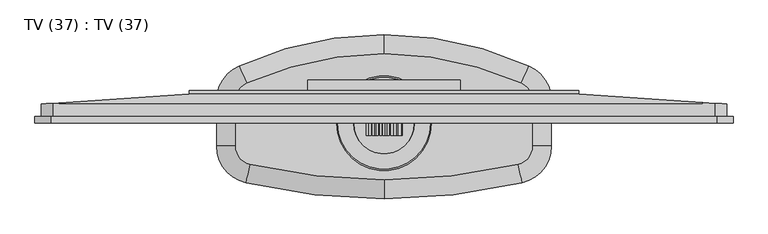
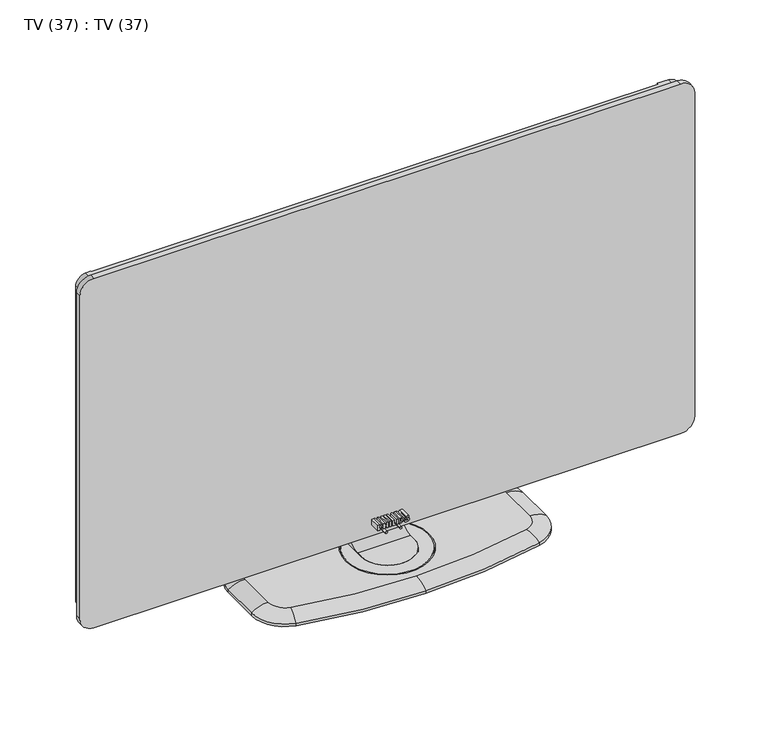
"""IFC4 building model written with IfcOpenShell, lengths in millimetres: furniture geometry, TV (37) : TV (37)."""

from ifc_helpers import new_model, si_unit, point, frame, frame_2d, origin, place, context, project, spatial, polyline, circle_curve, ellipse_curve, trimmed, segment, composite_curve, outline, extrude, source, transform, mapped, element, save
from ifc_brep_helpers import plane_surface, cylinder_surface, revolved_surface, advanced_brep


def tv_37_tv_37_55a44b14(model_context):
    return source(origin(), model_context, "Body", "SolidModel", [
        advanced_brep(
        [(47.5, 88.0, 133.1843541), (47.5, 88.0, 218.1843541), (47.5, 78.0, 218.1843541), (47.5, 78.0, 133.6678583), (47.5, 59.7827761, 41.2895959), (47.5, 32.0312094, 20.0814552), (47.5, 29.7558767, 20.0), (47.5, 18.8623336, 20.0), (47.5, 18.8623336, 10.0), (47.5, 44.5, 10.0), (47.5, 69.2193203, 37.9802704), (-47.5, 88.0, 133.1843541), (-47.5, 69.2193203, 37.9802704), (-47.5, 44.5, 10.0), (-47.5, 18.8623336, 10.0), (-47.5, 18.8623336, 20.0), (-47.5, 29.7558767, 20.0), (-47.5, 32.0312094, 20.0814552), (-47.5, 59.7827761, 41.2895959), (-47.5, 78.0, 133.6678583), (-47.5, 78.0, 218.1843541), (-47.5, 88.0, 218.1843541)],
        [
            (0, 1),
            (1, 2),
            (2, 3),
            (3, 4, circle_curve(frame((47.5, -252.8458142, 150.9261062), z_axis=(-1.0, 0.0, 0.0), x_axis=(0.0, 1.0, 0.0)), 331.2956382)),
            (4, 5, circle_curve(frame((47.5, 29.7558767, 51.8198052), z_axis=(-1.0, 0.0, 0.0), x_axis=(0.0, 1.0, 0.0)), 31.8198052)),
            (5, 6, circle_curve(frame((47.5, 29.7558767, 51.8198052), z_axis=(-1.0, 0.0, 0.0), x_axis=(0.0, 1.0, 0.0)), 31.8198052)),
            (6, 7),
            (7, 8),
            (8, 9),
            (9, 10, circle_curve(frame((47.5, 16.5507824, 59.6012298), z_axis=(1.0, 0.0, 0.0), x_axis=(0.0, 1.0, 0.0)), 56.9336523)),
            (10, 0, circle_curve(frame((47.5, -162.6973021, 133.1843541), z_axis=(1.0, 0.0, 0.0), x_axis=(0.0, 1.0, 0.0)), 250.6973021)),
            (11, 12, circle_curve(frame((-47.5, -162.6973021, 133.1843541), z_axis=(-1.0, 0.0, 0.0), x_axis=(0.0, 1.0, 0.0)), 250.6973021)),
            (12, 13, circle_curve(frame((-47.5, 16.5507824, 59.6012298), z_axis=(-1.0, 0.0, 0.0), x_axis=(0.0, 1.0, 0.0)), 56.9336523)),
            (13, 14),
            (14, 15),
            (15, 16),
            (16, 17, circle_curve(frame((-47.5, 29.7558767, 51.8198052), z_axis=(1.0, 0.0, 0.0), x_axis=(0.0, 1.0, 0.0)), 31.8198052)),
            (17, 18, circle_curve(frame((-47.5, 29.7558767, 51.8198052), z_axis=(1.0, 0.0, 0.0), x_axis=(0.0, 1.0, 0.0)), 31.8198052)),
            (18, 19, circle_curve(frame((-47.5, -252.8458142, 150.9261062), z_axis=(1.0, 0.0, 0.0), x_axis=(0.0, 1.0, 0.0)), 331.2956382)),
            (19, 20),
            (20, 21),
            (21, 11),
            (0, 11),
            (21, 1),
            (20, 2),
            (19, 3),
            (18, 4),
            (16, 6),
            (15, 7, circle_curve(frame((0.0, 18.8623336, 20.0), z_axis=(0.0, 0.0, 1.0), x_axis=(1.0, 0.0, 0.0)), 47.5)),
            (8, 14, circle_curve(frame((0.0, 18.8623336, 10.0), z_axis=(0.0, 0.0, -1.0), x_axis=(1.0, 0.0, 0.0)), 47.5)),
            (13, 9),
            (12, 10),
        ],
        [
            plane_surface(frame((47.5, 88.0, 393.1843541), z_axis=(1.0, 0.0, 0.0), x_axis=(0.0, 0.0, 1.0))),
            plane_surface(frame((-47.5, 88.0, 393.1843541), z_axis=(-1.0, 0.0, 0.0), x_axis=(0.0, 0.0, -1.0))),
            plane_surface(frame((47.5, 88.0, 133.1843541), z_axis=(0.0, 1.0, 0.0), x_axis=(-1.0, 0.0, 0.0))),
            plane_surface(frame((47.5, 88.0, 218.1843541), z_axis=(0.0, 0.0, 1.0), x_axis=(-1.0, 0.0, 0.0))),
            plane_surface(frame((47.5, 78.0, 218.1843541), z_axis=(0.0, -1.0, 0.0), x_axis=(-1.0, 0.0, 0.0))),
            revolved_surface(polyline([(-47.5, 78.44982399999998, 150.9261062), (47.5, 78.44982399999998, 150.9261062)]), (-47.5, -252.8458142, 150.9261062), (-1.0, 0.0, 0.0)),
            revolved_surface(polyline([(-47.5, 61.575681900000006, 51.8198052), (47.5, 61.575681900000006, 51.8198052)]), (-47.5, 29.7558767, 51.8198052), (-1.0, 0.0, 0.0)),
            plane_surface(frame((47.5, 29.7558767, 20.0), z_axis=(0.0, 0.0, 1.0), x_axis=(-1.0, 0.0, 0.0))),
            plane_surface(frame((47.5, 18.8623336, 10.0), z_axis=(0.0, 0.0, -1.0), x_axis=(-1.0, 0.0, 0.0))),
            cylinder_surface(frame((-47.5, 16.5507824, 59.6012298), z_axis=(1.0, 0.0, 0.0), x_axis=(0.0, 1.0, 0.0)), 56.9336523),
            cylinder_surface(frame((-47.5, -162.6973021, 133.1843541), z_axis=(1.0, 0.0, 0.0), x_axis=(0.0, 1.0, 0.0)), 250.6973021),
            cylinder_surface(frame((0.0, 18.8623336, 10.0), z_axis=(0.0, 0.0, 1.0), x_axis=(1.0, 0.0, 0.0)), 47.5),
        ],
        [
            (0, [[1, 2, 3, 4, 5, 6, 7, 8, 9, 10, 11]]),
            (1, [[12, 13, 14, 15, 16, 17, 18, 19, 20, 21, 22]]),
            (2, [[-1, 23, -22, 24]]),
            (3, [[-2, -24, -21, 25]]),
            (4, [[-3, -25, -20, 26]]),
            (5, [[-4, -26, -19, 27]]),
            (6, [[-27, -18, -17, 28, -6, -5]]),
            (7, [[-7, -28, -16, 29]]),
            (8, [[30, -14, 31, -9]]),
            (9, [[-10, -31, -13, 32]]),
            (10, [[-11, -32, -12, -23]]),
            (11, [[-29, -15, -30, -8]]),
        ],
    ),
        advanced_brep(
        [(-205.0, 88.7099995, 0.0), (-205.0, -47.2603519, 0.0), (-205.0, -47.2603519, 5.0), (-205.0, 88.7099995, 5.0), (-218.5849057, -74.9290034, 5.0), (-265.0, -16.4871491, 5.0), (-265.0, 55.9989024, 5.0), (-229.622384, 110.7139662, 5.0), (0.0, 160.0, 5.0), (229.622384, 110.7139662, 5.0), (265.0, 55.9989024, 5.0), (265.0, -16.4871491, 5.0), (218.5849057, -74.9290034, 5.0), (0.0, -100.0, 5.0), (0.0, -70.0, 5.0), (205.0, -47.2603519, 5.0), (205.0, 88.7099995, 5.0), (0.0, 130.0, 5.0), (-211.7924528, -45.7080763, 20.0), (0.0, -70.0, 20.0), (211.7924528, -45.7080763, 20.0), (235.0, -16.4871491, 20.0), (235.0, 55.9989024, 20.0), (217.311192, 83.3564343, 20.0), (0.0, 130.0, 20.0), (-217.311192, 83.3564343, 20.0), (-235.0, 55.9989024, 20.0), (-235.0, -16.4871491, 20.0), (75.0, 19.7558767, 20.0), (-75.0, 19.7558767, 20.0), (73.0, 19.7558767, 20.0), (-73.0, 19.7558767, 20.0), (48.0, 19.7558767, 20.0), (-48.0, 19.7558767, 20.0), (-48.0, 59.7558767, 20.0), (48.0, 59.7558767, 20.0), (205.0, -47.2603519, 0.0), (205.0, 88.7099995, 0.0), (0.0, 130.0, 0.0), (0.0, -70.0, 0.0), (-218.5849057, -74.9290034, 10.0), (0.0, -100.0, 10.0), (-265.0, -16.4871491, 10.0), (-265.0, 55.9989024, 10.0), (-229.622384, 110.7139662, 10.0), (0.0, 160.0, 10.0), (218.5849057, -74.9290034, 10.0), (265.0, -16.4871491, 10.0), (265.0, 55.9989024, 10.0), (229.622384, 110.7139662, 10.0), (-75.0, 19.7558767, 10.0), (75.0, 19.7558767, 10.0), (-73.0, 19.7558767, 10.0), (73.0, 19.7558767, 10.0), (48.0, 19.7558767, 10.0), (48.0, 59.7558767, 10.0), (-48.0, 59.7558767, 10.0), (-48.0, 19.7558767, 10.0)],
        [
            (0, 1),
            (1, 2),
            (2, 3),
            (3, 0),
            (4, 5, circle_curve(frame((-205.0, -16.4871491, 5.0), z_axis=(0.0, 0.0, -1.0), x_axis=(-0.22641509433980192, -0.9740309055954531, 0.0)), 60.0)),
            (5, 6),
            (6, 7, circle_curve(frame((-205.0, 55.9989024, 5.0), z_axis=(0.0, 0.0, -1.0), x_axis=(-1.0, 0.0, 0.0)), 60.0)),
            (7, 8, circle_curve(frame((0.0, -399.5454545, 5.0), z_axis=(0.0, 0.0, -1.0), x_axis=(-0.41037306642402943, 0.911917730035851, 0.0)), 559.5454545)),
            (8, 9, circle_curve(frame((0.0, -399.5454545, 5.0), z_axis=(0.0, 0.0, -1.0), x_axis=(0.41037306642402943, 0.911917730035851, 0.0)), 559.5454545)),
            (9, 10, circle_curve(frame((205.0, 55.9989024, 5.0), z_axis=(0.0, 0.0, -1.0), x_axis=(1.0, 0.0, 0.0)), 60.0)),
            (10, 11),
            (11, 12, circle_curve(frame((205.0, -16.4871491, 5.0), z_axis=(0.0, 0.0, -1.0), x_axis=(0.22641509433980192, -0.9740309055954531, 0.0)), 60.0)),
            (12, 13, circle_curve(frame((0.0, 865.4166667, 5.0), z_axis=(0.0, 0.0, -1.0), x_axis=(0.0, -1.0, 0.0)), 965.4166667)),
            (13, 4, circle_curve(frame((0.0, 865.4166667, 5.0), z_axis=(0.0, 0.0, -1.0), x_axis=(0.0, -1.0, 0.0)), 965.4166667)),
            (2, 14, circle_curve(frame((0.0, 865.4166667, 5.0), z_axis=(0.0, 0.0, 1.0), x_axis=(0.0, -1.0, 0.0)), 935.4166667)),
            (14, 15, circle_curve(frame((0.0, 865.4166667, 5.0), z_axis=(0.0, 0.0, 1.0), x_axis=(0.0, -1.0, 0.0)), 935.4166667)),
            (15, 16),
            (16, 17, circle_curve(frame((0.0, -399.5454545, 5.0), z_axis=(0.0, 0.0, 1.0), x_axis=(0.41037306642402943, 0.911917730035851, 0.0)), 529.5454545)),
            (17, 3, circle_curve(frame((0.0, -399.5454545, 5.0), z_axis=(0.0, 0.0, 1.0), x_axis=(-0.41037306642402943, 0.911917730035851, 0.0)), 529.5454545)),
            (18, 19, circle_curve(frame((0.0, 865.4166667, 20.0), z_axis=(0.0, 0.0, 1.0), x_axis=(0.0, -1.0, 0.0)), 935.4166667)),
            (19, 20, circle_curve(frame((0.0, 865.4166667, 20.0), z_axis=(0.0, 0.0, 1.0), x_axis=(0.0, -1.0, 0.0)), 935.4166667)),
            (20, 21, circle_curve(frame((205.0, -16.4871491, 20.0), z_axis=(0.0, 0.0, 1.0), x_axis=(0.22641509433980192, -0.9740309055954531, 0.0)), 30.0)),
            (21, 22),
            (22, 23, circle_curve(frame((205.0, 55.9989024, 20.0), z_axis=(0.0, 0.0, 1.0), x_axis=(1.0, 0.0, 0.0)), 30.0)),
            (23, 24, circle_curve(frame((0.0, -399.5454545, 20.0), z_axis=(0.0, 0.0, 1.0), x_axis=(0.41037306642402943, 0.911917730035851, 0.0)), 529.5454545)),
            (24, 25, circle_curve(frame((0.0, -399.5454545, 20.0), z_axis=(0.0, 0.0, 1.0), x_axis=(-0.41037306642402943, 0.911917730035851, 0.0)), 529.5454545)),
            (25, 26, circle_curve(frame((-205.0, 55.9989024, 20.0), z_axis=(0.0, 0.0, 1.0), x_axis=(-1.0, 0.0, 0.0)), 30.0)),
            (26, 27),
            (27, 18, circle_curve(frame((-205.0, -16.4871491, 20.0), z_axis=(0.0, 0.0, 1.0), x_axis=(-0.22641509433980192, -0.9740309055954531, 0.0)), 30.0)),
            (28, 29, circle_curve(frame((0.0, 19.7558767, 20.0), z_axis=(0.0, 0.0, -1.0), x_axis=(1.0, 0.0, 0.0)), 75.0)),
            (29, 28, circle_curve(frame((0.0, 19.7558767, 20.0), z_axis=(0.0, 0.0, -1.0), x_axis=(1.0, 0.0, 0.0)), 75.0)),
            (30, 31, circle_curve(frame((0.0, 19.7558767, 20.0), z_axis=(0.0, 0.0, 1.0), x_axis=(1.0, 0.0, 0.0)), 73.0)),
            (31, 30, circle_curve(frame((0.0, 19.7558767, 20.0), z_axis=(0.0, 0.0, 1.0), x_axis=(1.0, 0.0, 0.0)), 73.0)),
            (32, 33, circle_curve(frame((0.0, 19.7558767, 20.0), z_axis=(0.0, 0.0, -1.0), x_axis=(1.0, 0.0, 0.0)), 48.0)),
            (33, 34),
            (34, 35),
            (35, 32),
            (15, 36),
            (36, 37),
            (37, 16),
            (0, 38, circle_curve(frame((0.0, -399.5454545, 0.0), z_axis=(0.0, 0.0, -1.0), x_axis=(-0.41037306642402943, 0.911917730035851, 0.0)), 529.5454545)),
            (38, 37, circle_curve(frame((0.0, -399.5454545, 0.0), z_axis=(0.0, 0.0, -1.0), x_axis=(0.41037306642402943, 0.911917730035851, 0.0)), 529.5454545)),
            (36, 39, circle_curve(frame((0.0, 865.4166667, 0.0), z_axis=(0.0, 0.0, -1.0), x_axis=(0.0, -1.0, 0.0)), 935.4166667)),
            (39, 1, circle_curve(frame((0.0, 865.4166667, 0.0), z_axis=(0.0, 0.0, -1.0), x_axis=(0.0, -1.0, 0.0)), 935.4166667)),
            (18, 40, circle_curve(frame((-211.7924528, -45.7080763, -30.0), z_axis=(0.9740309055954945, -0.22641509433962395, 0.0), x_axis=(0.22641509433962395, 0.9740309055954945, 0.0)), 50.0)),
            (40, 41, circle_curve(frame((0.0, 865.4166667, 10.0), z_axis=(0.0, 0.0, 1.0), x_axis=(0.0, -1.0, 0.0)), 965.4166667)),
            (41, 19, circle_curve(frame((0.0, -70.0, -30.0), z_axis=(-1.0, 0.0, 0.0), x_axis=(0.0, 1.0, 0.0)), 50.0)),
            (39, 14),
            (40, 4),
            (13, 41),
            (27, 42, circle_curve(frame((-235.0, -16.4871491, -30.0), z_axis=(0.0, -1.0, 0.0), x_axis=(1.0, 0.0, 0.0)), 50.0)),
            (42, 40, circle_curve(frame((-205.0, -16.4871491, 10.0), z_axis=(0.0, 0.0, 1.0), x_axis=(-0.22641509433980192, -0.9740309055954531, 0.0)), 60.0)),
            (42, 5),
            (26, 43, circle_curve(frame((-235.0, 55.9989024, -30.0), z_axis=(0.0, -1.0, 0.0), x_axis=(1.0, 0.0, 0.0)), 50.0)),
            (43, 42),
            (43, 6),
            (25, 44, circle_curve(frame((-217.311192, 83.3564343, -30.0), z_axis=(-0.911917730035806, -0.41037306642412946, 0.0), x_axis=(0.41037306642412946, -0.911917730035806, 0.0)), 50.0)),
            (44, 43, circle_curve(frame((-205.0, 55.9989024, 10.0), z_axis=(0.0, 0.0, 1.0), x_axis=(-1.0, 0.0, 0.0)), 60.0)),
            (44, 7),
            (24, 45, circle_curve(frame((0.0, 130.0, -30.0), z_axis=(-1.0, 0.0, 0.0), x_axis=(0.0, -1.0, 0.0)), 50.0)),
            (45, 44, circle_curve(frame((0.0, -399.5454545, 10.0), z_axis=(0.0, 0.0, 1.0), x_axis=(-0.41037306642402943, 0.911917730035851, 0.0)), 559.5454545)),
            (17, 38),
            (45, 8),
            (12, 46),
            (46, 41, circle_curve(frame((0.0, 865.4166667, 10.0), z_axis=(0.0, 0.0, -1.0), x_axis=(0.0, -1.0, 0.0)), 965.4166667)),
            (46, 20, circle_curve(frame((211.7924528, -45.7080763, -30.0), z_axis=(-0.9740309055954932, -0.22641509433962945, 0.0), x_axis=(-0.22641509433962945, 0.9740309055954932, 0.0)), 50.0)),
            (11, 47),
            (47, 46, circle_curve(frame((205.0, -16.4871491, 10.0), z_axis=(0.0, 0.0, -1.0), x_axis=(0.22641509433980192, -0.9740309055954531, 0.0)), 60.0)),
            (47, 21, circle_curve(frame((235.0, -16.4871491, -30.0), z_axis=(0.0, -1.0, 0.0), x_axis=(-1.0, 0.0, 0.0)), 50.0)),
            (10, 48),
            (48, 47),
            (48, 22, circle_curve(frame((235.0, 55.9989024, -30.0), z_axis=(0.0, -1.0, 0.0), x_axis=(-1.0, 0.0, 0.0)), 50.0)),
            (9, 49),
            (49, 48, circle_curve(frame((205.0, 55.9989024, 10.0), z_axis=(0.0, 0.0, -1.0), x_axis=(1.0, 0.0, 0.0)), 60.0)),
            (49, 23, circle_curve(frame((217.311192, 83.3564343, -30.0), z_axis=(0.9119177300358283, -0.41037306642407984, 0.0), x_axis=(-0.41037306642407984, -0.9119177300358283, 0.0)), 50.0)),
            (45, 49, circle_curve(frame((0.0, -399.5454545, 10.0), z_axis=(0.0, 0.0, -1.0), x_axis=(0.41037306642402943, 0.911917730035851, 0.0)), 559.5454545)),
            (50, 51, circle_curve(frame((0.0, 19.7558767, 10.0), z_axis=(0.0, 0.0, 1.0), x_axis=(1.0, 0.0, 0.0)), 75.0)),
            (51, 50, circle_curve(frame((0.0, 19.7558767, 10.0), z_axis=(0.0, 0.0, 1.0), x_axis=(1.0, 0.0, 0.0)), 75.0)),
            (52, 53, circle_curve(frame((0.0, 19.7558767, 10.0), z_axis=(0.0, 0.0, -1.0), x_axis=(1.0, 0.0, 0.0)), 73.0)),
            (53, 52, circle_curve(frame((0.0, 19.7558767, 10.0), z_axis=(0.0, 0.0, -1.0), x_axis=(1.0, 0.0, 0.0)), 73.0)),
            (54, 55),
            (55, 56),
            (56, 57),
            (57, 54, circle_curve(frame((0.0, 19.7558767, 10.0), z_axis=(0.0, 0.0, 1.0), x_axis=(1.0, 0.0, 0.0)), 48.0)),
            (50, 29),
            (28, 51),
            (52, 31),
            (30, 53),
            (54, 32),
            (35, 55),
            (34, 56),
            (33, 57),
        ],
        [
            plane_surface(frame((-205.0, 190.0, 0.0), z_axis=(-1.0, 0.0, 0.0), x_axis=(0.0, -1.0, 0.0))),
            plane_surface(frame((-205.0, 190.0, 5.0), z_axis=(0.0, 0.0, -1.0), x_axis=(0.0, -1.0, 0.0))),
            plane_surface(frame((-295.0, 190.0, 20.0), z_axis=(0.0, 0.0, 1.0), x_axis=(0.0, -1.0, 0.0))),
            plane_surface(frame((205.0, 190.0, 5.0), z_axis=(1.0, 0.0, 0.0), x_axis=(0.0, -1.0, 0.0))),
            plane_surface(frame((205.0, 190.0, 0.0), z_axis=(0.0, 0.0, -1.0), x_axis=(0.0, -1.0, 0.0))),
            revolved_surface(trimmed(ellipse_curve(frame((0.0, -70.0, -30.0), z_axis=(1.0, 0.0, 0.0), x_axis=(0.0, 1.0, 0.0)), 50.0, 50.0), [point((0.0, -70.0, 20.0))], [point((0.0, -100.0, 10.0))], True, "CARTESIAN"), (0.0, 865.4166667, 0.0), (0.0, 0.0, -1.0)),
            cylinder_surface(frame((0.0, 865.4166667, 0.0), z_axis=(0.0, 0.0, -1.0), x_axis=(0.0, -1.0, 0.0)), 935.4166667),
            cylinder_surface(frame((0.0, 865.4166667, 0.0), z_axis=(0.0, 0.0, -1.0), x_axis=(0.0, -1.0, 0.0)), 965.4166667),
            revolved_surface(trimmed(ellipse_curve(frame((-211.7924528, -45.7080763, -30.0), z_axis=(0.9740309055954531, -0.22641509433980195, 0.0), x_axis=(0.22641509433980195, 0.9740309055954531, 0.0)), 50.0, 50.0), [point((-211.7924528, -45.7080763, 20.0))], [point((-218.5849057, -74.9290034, 10.0))], True, "CARTESIAN"), (-205.0, -16.4871491, 0.0), (0.0, 0.0, -1.0)),
            cylinder_surface(frame((-205.0, -16.4871491, 0.0), z_axis=(0.0, 0.0, -1.0), x_axis=(-0.22641509433980192, -0.9740309055954531, 0.0)), 60.0),
            cylinder_surface(frame((-235.0, -16.4871491, -30.0), z_axis=(0.0, 1.0, 0.0), x_axis=(1.0, 0.0, 0.0)), 50.0),
            plane_surface(frame((-265.0, -16.4871491, 5.0), z_axis=(-1.0, 0.0, 0.0), x_axis=(0.0, 1.0, 0.0))),
            revolved_surface(trimmed(ellipse_curve(frame((-235.0, 55.9989024, -30.0), z_axis=(0.0, -1.0, 0.0), x_axis=(1.0, 0.0, 0.0)), 50.0, 50.0), [point((-235.0, 55.9989024, 20.0))], [point((-265.0, 55.9989024, 10.0))], True, "CARTESIAN"), (-205.0, 55.9989024, 0.0), (0.0, 0.0, -1.0)),
            cylinder_surface(frame((-205.0, 55.9989024, 0.0), z_axis=(0.0, 0.0, -1.0), x_axis=(-1.0, 0.0, 0.0)), 60.0),
            revolved_surface(trimmed(ellipse_curve(frame((-217.311192, 83.3564343, -30.0), z_axis=(-0.911917730035851, -0.4103730664240294, 0.0), x_axis=(0.4103730664240294, -0.911917730035851, 0.0)), 50.0, 50.0), [point((-217.311192, 83.3564343, 20.0))], [point((-229.622384, 110.7139662, 10.0))], True, "CARTESIAN"), (0.0, -399.5454545, 0.0), (0.0, 0.0, -1.0)),
            cylinder_surface(frame((0.0, -399.5454545, 0.0), z_axis=(0.0, 0.0, -1.0), x_axis=(-0.41037306642402943, 0.911917730035851, 0.0)), 529.5454545),
            cylinder_surface(frame((0.0, -399.5454545, 0.0), z_axis=(0.0, 0.0, -1.0), x_axis=(-0.41037306642402943, 0.911917730035851, 0.0)), 559.5454545),
            cylinder_surface(frame((0.0, 865.4166667, 0.0), z_axis=(0.0, 0.0, 1.0), x_axis=(0.0, -1.0, 0.0)), 965.4166667),
            cylinder_surface(frame((0.0, 865.4166667, 0.0), z_axis=(0.0, 0.0, 1.0), x_axis=(0.0, -1.0, 0.0)), 935.4166667),
            revolved_surface(trimmed(ellipse_curve(frame((0.0, -70.0, -30.0), z_axis=(-1.0, 0.0, 0.0), x_axis=(0.0, 1.0, 0.0)), 50.0, 50.0), [point((0.0, -100.0, 10.0))], [point((0.0, -70.0, 20.0))], True, "CARTESIAN"), (0.0, 865.4166667, 0.0), (0.0, 0.0, 1.0)),
            cylinder_surface(frame((205.0, -16.4871491, 0.0), z_axis=(0.0, 0.0, 1.0), x_axis=(0.22641509433980192, -0.9740309055954531, 0.0)), 60.0),
            revolved_surface(trimmed(ellipse_curve(frame((211.7924528, -45.7080763, -30.0), z_axis=(-0.9740309055954531, -0.22641509433980195, 0.0), x_axis=(-0.22641509433980195, 0.9740309055954531, 0.0)), 50.0, 50.0), [point((218.5849057, -74.9290034, 10.0))], [point((211.7924528, -45.7080763, 20.0))], True, "CARTESIAN"), (205.0, -16.4871491, 0.0), (0.0, 0.0, 1.0)),
            plane_surface(frame((265.0, -16.4871491, 10.0), z_axis=(1.0, 0.0, 0.0), x_axis=(0.0, 1.0, 0.0))),
            cylinder_surface(frame((235.0, -16.4871491, -30.0), z_axis=(0.0, 1.0, 0.0), x_axis=(-1.0, 0.0, 0.0)), 50.0),
            cylinder_surface(frame((205.0, 55.9989024, 0.0), z_axis=(0.0, 0.0, 1.0), x_axis=(1.0, 0.0, 0.0)), 60.0),
            revolved_surface(trimmed(ellipse_curve(frame((235.0, 55.9989024, -30.0), z_axis=(0.0, -1.0, 0.0), x_axis=(-1.0, 0.0, 0.0)), 50.0, 50.0), [point((265.0, 55.9989024, 10.0))], [point((235.0, 55.9989024, 20.0))], True, "CARTESIAN"), (205.0, 55.9989024, 0.0), (0.0, 0.0, 1.0)),
            cylinder_surface(frame((0.0, -399.5454545, 0.0), z_axis=(0.0, 0.0, 1.0), x_axis=(0.41037306642402943, 0.911917730035851, 0.0)), 559.5454545),
            cylinder_surface(frame((0.0, -399.5454545, 0.0), z_axis=(0.0, 0.0, 1.0), x_axis=(0.41037306642402943, 0.911917730035851, 0.0)), 529.5454545),
            revolved_surface(trimmed(ellipse_curve(frame((217.311192, 83.3564343, -30.0), z_axis=(0.911917730035851, -0.4103730664240294, 0.0), x_axis=(-0.4103730664240294, -0.911917730035851, 0.0)), 50.0, 50.0), [point((229.622384, 110.7139662, 10.0))], [point((217.311192, 83.3564343, 20.0))], True, "CARTESIAN"), (0.0, -399.5454545, 0.0), (0.0, 0.0, 1.0)),
            plane_surface(frame((75.0, 19.7558767, 10.0), z_axis=(0.0, 0.0, 1.0), x_axis=(0.0, -1.0, 0.0))),
            revolved_surface(polyline([(75.0, 19.7558767, 20.0), (75.0, 19.7558767, 10.0)]), (0.0, 19.7558767, 10.0), (0.0, 0.0, 1.0)),
            cylinder_surface(frame((0.0, 19.7558767, 0.0), z_axis=(0.0, 0.0, -1.0), x_axis=(1.0, 0.0, 0.0)), 73.0),
            plane_surface(frame((48.0, 19.7558767, 20.0), z_axis=(-1.0, 0.0, 0.0), x_axis=(0.0, 0.0, -1.0))),
            plane_surface(frame((48.0, 59.7558767, 20.0), z_axis=(0.0, -1.0, 0.0), x_axis=(0.0, 0.0, -1.0))),
            plane_surface(frame((-48.0, 59.7558767, 20.0), z_axis=(1.0, 0.0, 0.0), x_axis=(0.0, 0.0, -1.0))),
            revolved_surface(polyline([(48.0, 19.7558767, 20.0), (48.0, 19.7558767, 10.0)]), (0.0, 19.7558767, 0.0), (0.0, 0.0, 1.0)),
        ],
        [
            (0, [[1, 2, 3, 4]]),
            (1, [[5, 6, 7, 8, 9, 10, 11, 12, 13, 14], [15, 16, 17, 18, 19, -3]]),
            (2, [[20, 21, 22, 23, 24, 25, 26, 27, 28, 29], [30, 31]]),
            (2, [[32, 33], [34, 35, 36, 37]]),
            (3, [[-17, 38, 39, 40]]),
            (4, [[-1, 41, 42, -39, 43, 44]]),
            (5, [[45, 46, 47, -20]]),
            (6, [[-15, -2, -44, 48]]),
            (7, [[-46, 49, -14, 50]]),
            (8, [[-45, -29, 51, 52]]),
            (9, [[-49, -52, 53, -5]]),
            (10, [[-51, -28, 54, 55]]),
            (11, [[-53, -55, 56, -6]]),
            (12, [[-54, -27, 57, 58]]),
            (13, [[-56, -58, 59, -7]]),
            (14, [[-57, -26, 60, 61]]),
            (15, [[-19, 62, -41, -4]]),
            (16, [[-59, -61, 63, -8]]),
            (17, [[64, 65, -50, -13]]),
            (18, [[-16, -48, -43, -38]]),
            (19, [[-65, 66, -21, -47]]),
            (20, [[-64, -12, 67, 68]]),
            (21, [[-66, -68, 69, -22]]),
            (22, [[-67, -11, 70, 71]]),
            (23, [[-69, -71, 72, -23]]),
            (24, [[-70, -10, 73, 74]]),
            (25, [[-72, -74, 75, -24]]),
            (26, [[-73, -9, -63, 76]]),
            (27, [[-18, -40, -42, -62]]),
            (28, [[-75, -76, -60, -25]]),
            (29, [[77, 78], [79, 80]]),
            (29, [[81, 82, 83, 84]]),
            (30, [[-77, 85, -30, 86]]),
            (30, [[-78, -86, -31, -85]]),
            (31, [[-79, 87, -32, 88]]),
            (31, [[-80, -88, -33, -87]]),
            (32, [[-81, 89, -37, 90]]),
            (33, [[-82, -90, -36, 91]]),
            (34, [[-83, -91, -35, 92]]),
            (35, [[-84, -92, -34, -89]]),
        ],
    ),
        advanced_brep(
        [(-120.5724482, 88.0, 218.1843541), (-120.5724482, 88.0, 453.1843541), (120.5724482, 88.0, 453.1843541), (120.5724482, 88.0, 218.1843541), (-525.0, 30.0, 707.0), (-543.0, 30.0, 689.0), (-543.0, 30.0, 93.0), (-525.0, 30.0, 75.0), (-515.0, 30.0, 75.0), (505.0, 30.0, 75.0), (525.0, 30.0, 75.0), (543.0, 30.0, 93.0), (543.0, 30.0, 689.0), (525.0, 30.0, 707.0), (505.0, 30.0, 707.0), (-515.0, 30.0, 707.0), (543.0, 50.0, 689.0), (525.0, 51.2586826, 707.0), (543.0, 50.0, 93.0), (525.0, 51.2586826, 75.0), (-525.0, 51.2586826, 75.0), (-515.0, 51.9579507, 75.0), (-515.0, 50.0, 75.0), (505.0, 50.0, 75.0), (505.0, 52.6572189, 75.0), (-543.0, 50.0, 93.0), (-543.0, 50.0, 689.0), (-525.0, 51.2586826, 707.0), (505.0, 52.6572189, 707.0), (505.0, 50.0, 707.0), (-515.0, 50.0, 707.0), (-515.0, 51.9579507, 707.0), (-515.0, 51.9579507, 682.0590831), (-308.5724482, 66.3927713, 498.1843541), (-308.5724482, 66.3927713, 168.1843541), (-515.0, 51.9579507, 86.1299286), (-308.5724482, 71.3927713, 498.1843541), (-308.5724482, 71.3927713, 168.1843541), (308.5724482, 71.3927713, 498.1843541), (308.5724482, 71.3927713, 168.1843541), (-120.5724482, 71.3927713, 218.1843541), (120.5724482, 71.3927713, 218.1843541), (120.5724482, 71.3927713, 453.1843541), (-120.5724482, 71.3927713, 453.1843541), (308.5724482, 66.3927713, 498.1843541), (308.5724482, 66.3927713, 168.1843541), (505.0, 52.6572189, 90.1049031), (505.0, 52.6572189, 673.1516128)],
        [
            (0, 1),
            (1, 2),
            (2, 3),
            (3, 0),
            (4, 5, circle_curve(frame((-525.0, 30.0, 689.0), z_axis=(0.0, -1.0, 0.0), x_axis=(1.0, 0.0, 0.0)), 18.0)),
            (5, 6),
            (6, 7, circle_curve(frame((-525.0, 30.0, 93.0), z_axis=(0.0, -1.0, 0.0), x_axis=(1.0, 0.0, 0.0)), 18.0)),
            (7, 8),
            (8, 9),
            (9, 10),
            (10, 11, circle_curve(frame((525.0, 30.0, 93.0), z_axis=(0.0, -1.0, 0.0), x_axis=(1.0, 0.0, 0.0)), 18.0)),
            (11, 12),
            (12, 13, circle_curve(frame((525.0, 30.0, 689.0), z_axis=(0.0, -1.0, 0.0), x_axis=(1.0, 0.0, 0.0)), 18.0)),
            (13, 14),
            (14, 15),
            (15, 4),
            (12, 16),
            (16, 17, ellipse_curve(frame((525.0, 51.2586826, 689.0), z_axis=(-0.06975647374412541, -0.9975640502598243, 0.0), x_axis=(-0.9975640502598244, 0.06975647374412326, 0.0)), 18.0439542, 18.0)),
            (17, 13),
            (11, 18),
            (18, 16),
            (10, 19),
            (19, 18, ellipse_curve(frame((525.0, 51.2586826, 93.0), z_axis=(-0.06975647374412541, -0.9975640502598243, 0.0), x_axis=(-0.9975640502598244, 0.06975647374412326, 0.0)), 18.0439542, 18.0)),
            (7, 20),
            (20, 21),
            (21, 22),
            (22, 23),
            (23, 24),
            (24, 19),
            (6, 25),
            (25, 20, ellipse_curve(frame((-525.0, 51.2586826, 93.0), z_axis=(0.06975647374412541, -0.9975640502598243, 0.0), x_axis=(0.9975640502598244, 0.06975647374412326, 0.0)), 18.0439542, 18.0)),
            (5, 26),
            (26, 25),
            (4, 27),
            (27, 26, ellipse_curve(frame((-525.0, 51.2586826, 689.0), z_axis=(0.06975647374412541, -0.9975640502598243, 0.0), x_axis=(0.9975640502598244, 0.06975647374412326, 0.0)), 18.0439542, 18.0)),
            (17, 28),
            (28, 29),
            (29, 30),
            (30, 31),
            (31, 27),
            (31, 32),
            (32, 33),
            (33, 34),
            (34, 35),
            (35, 21),
            (33, 36),
            (36, 37),
            (37, 34),
            (36, 38),
            (38, 39),
            (39, 37),
            (40, 41),
            (41, 42),
            (42, 43),
            (43, 40),
            (0, 40),
            (43, 1),
            (2, 42),
            (41, 3),
            (38, 44),
            (44, 45),
            (45, 39),
            (24, 46),
            (46, 45),
            (44, 47),
            (47, 28),
            (23, 46),
            (47, 29),
            (30, 32),
            (35, 22),
            (44, 33),
            (45, 34),
        ],
        [
            plane_surface(frame((543.0, 88.0, 689.0), z_axis=(0.0, 1.0, 0.0), x_axis=(0.0, 0.0, -1.0))),
            plane_surface(frame((543.0, 30.0, 689.0), z_axis=(0.0, -1.0, 0.0), x_axis=(0.0, 0.0, 1.0))),
            cylinder_surface(frame((525.0, 30.0, 689.0), z_axis=(0.0, 1.0, 0.0), x_axis=(1.0, 0.0, 0.0)), 18.0),
            plane_surface(frame((543.0, 88.0, 689.0), z_axis=(1.0, 0.0, 0.0), x_axis=(0.0, -1.0, 0.0))),
            cylinder_surface(frame((525.0, 30.0, 93.0), z_axis=(0.0, 1.0, 0.0), x_axis=(1.0, 0.0, 0.0)), 18.0),
            plane_surface(frame((525.0, 88.0, 75.0), z_axis=(0.0, 0.0, -1.0), x_axis=(0.0, -1.0, 0.0))),
            cylinder_surface(frame((-525.0, 30.0, 93.0), z_axis=(0.0, 1.0, 0.0), x_axis=(1.0, 0.0, 0.0)), 18.0),
            plane_surface(frame((-543.0, 88.0, 93.0), z_axis=(-1.0, 0.0, 0.0), x_axis=(0.0, -1.0, 0.0))),
            cylinder_surface(frame((-525.0, 30.0, 689.0), z_axis=(0.0, 1.0, 0.0), x_axis=(1.0, 0.0, 0.0)), 18.0),
            plane_surface(frame((-525.0, 88.0, 707.0), z_axis=(0.0, 0.0, 1.0), x_axis=(0.0, -1.0, 0.0))),
            plane_surface(frame((-543.0, 50.0, 735.0), z_axis=(-0.06975647374412541, 0.9975640502598243, 0.0), x_axis=(0.0, 0.0, -1.0))),
            plane_surface(frame((-308.5724482, 66.3927713, 735.0), z_axis=(-1.0, 0.0, 0.0), x_axis=(0.0, 0.0, -1.0))),
            plane_surface(frame((-308.5724482, 71.3927713, 735.0), z_axis=(0.0, 1.0, 0.0), x_axis=(0.0, 0.0, -1.0))),
            plane_surface(frame((-120.5724482, 71.3927713, 735.0), z_axis=(-1.0, 0.0, 0.0), x_axis=(0.0, 0.0, -1.0))),
            plane_surface(frame((120.5724482, 88.0, 735.0), z_axis=(1.0, 0.0, 0.0), x_axis=(0.0, 0.0, -1.0))),
            plane_surface(frame((308.5724482, 71.3927713, 735.0), z_axis=(1.0, 0.0, 0.0), x_axis=(0.0, 0.0, -1.0))),
            plane_surface(frame((308.5724482, 66.3927713, 735.0), z_axis=(0.06975647374412541, 0.9975640502598243, 0.0), x_axis=(0.0, 0.0, -1.0))),
            plane_surface(frame((505.0, 50.0, 707.0), z_axis=(-1.0, 0.0, 0.0), x_axis=(0.0, 0.07826276994630116, -0.9969327654562932))),
            plane_surface(frame((-515.0, 50.0, 707.0), z_axis=(1.0, 0.0, 0.0), x_axis=(0.0, -0.07826276994630116, 0.9969327654562932))),
            plane_surface(frame((505.0, 50.0, 707.0), z_axis=(0.0, 0.9969327654562932, 0.07826276994630116), x_axis=(-1.0, 0.0, 0.0))),
            plane_surface(frame((505.0, 66.3927713, 498.1843541), z_axis=(0.0, 0.0, 1.0), x_axis=(-1.0, 0.0, 0.0))),
            plane_surface(frame((505.0, 71.3927713, 453.1843541), z_axis=(0.0, 0.0, 1.0), x_axis=(-1.0, 0.0, 0.0))),
            plane_surface(frame((505.0, 88.0, 218.1843541), z_axis=(0.0, 0.0, -1.0), x_axis=(-1.0, 0.0, 0.0))),
            plane_surface(frame((505.0, 71.3927713, 168.1843541), z_axis=(0.0, 0.0, -1.0), x_axis=(-1.0, 0.0, 0.0))),
            plane_surface(frame((505.0, 66.3927713, 168.1843541), z_axis=(0.0, 0.9848766187169472, -0.17325716696481355), x_axis=(-1.0, 0.0, 0.0))),
        ],
        [
            (0, [[1, 2, 3, 4]]),
            (1, [[5, 6, 7, 8, 9, 10, 11, 12, 13, 14, 15, 16]]),
            (2, [[-13, 17, 18, 19]]),
            (3, [[-12, 20, 21, -17]]),
            (4, [[-11, 22, 23, -20]]),
            (5, [[-22, -10, -9, -8, 24, 25, 26, 27, 28, 29]]),
            (6, [[-7, 30, 31, -24]]),
            (7, [[-6, 32, 33, -30]]),
            (8, [[-5, 34, 35, -32]]),
            (9, [[-19, 36, 37, 38, 39, 40, -34, -16, -15, -14]]),
            (10, [[-31, -33, -35, -40, 41, 42, 43, 44, 45, -25]]),
            (11, [[-43, 46, 47, 48]]),
            (12, [[-47, 49, 50, 51], [52, 53, 54, 55]]),
            (13, [[-1, 56, -55, 57]]),
            (14, [[-3, 58, -53, 59]]),
            (15, [[-50, 60, 61, 62]]),
            (16, [[-18, -21, -23, -29, 63, 64, -61, 65, 66, -36]]),
            (17, [[67, -63, -28]]),
            (17, [[68, -37, -66]]),
            (18, [[69, -41, -39]]),
            (18, [[70, -26, -45]]),
            (19, [[71, -42, -69, -38, -68, -65]]),
            (20, [[-49, -46, -71, -60]]),
            (21, [[-54, -58, -2, -57]]),
            (22, [[-52, -56, -4, -59]]),
            (23, [[-51, -62, 72, -48]]),
            (24, [[-72, -64, -67, -27, -70, -44]]),
        ],
    ),
        extrude(outline(composite_curve([segment(polyline([(717.0, 528.0), (717.0, -528.0)]), True, "CONTINUOUS"), segment(trimmed(circle_curve(frame_2d((692.0, -528.0)), 25.0), [point((717.0, -528.0))], [point((692.0, -553.0))], False, "CARTESIAN"), True, "CONTINUOUS"), segment(polyline([(692.0, -553.0), (77.0, -553.0)]), True, "CONTINUOUS"), segment(trimmed(circle_curve(frame_2d((77.0, -528.0)), 25.0), [point((77.0, -553.0))], [point((52.0, -528.0))], False, "CARTESIAN"), True, "CONTINUOUS"), segment(polyline([(52.0, -528.0), (52.0, 528.0)]), True, "CONTINUOUS"), segment(trimmed(circle_curve(frame_2d((77.0, 528.0)), 25.0), [point((52.0, 528.0))], [point((77.0, 553.0))], False, "CARTESIAN"), True, "CONTINUOUS"), segment(polyline([(77.0, 553.0), (692.0, 553.0)]), True, "CONTINUOUS"), segment(trimmed(circle_curve(frame_2d((692.0, 528.0)), 25.0), [point((692.0, 553.0))], [point((717.0, 528.0))], False, "CARTESIAN"), True, "CONTINUOUS")], self_intersect=False)), frame((0.0, 20.0, 0.0), z_axis=(0.0, 1.0, 0.0), x_axis=(0.0, 0.0, 1.0)), (0.0, 0.0, 1.0), 10.0),
        extrude(outline(composite_curve([segment(polyline([(73.6143863, -28.3208351), (73.6143863, -25.3881417), (75.713327, -25.3881417), (75.713327, -23.8490711)]), True, "CONTINUOUS"), segment(trimmed(circle_curve(frame_2d((79.6638566, -23.8490711)), 3.9505297), [point((75.713327, -23.8490711))], [point((83.6143863, -23.8490711))], False, "CARTESIAN"), True, "CONTINUOUS"), segment(polyline([(83.6143863, -23.8490711), (83.6143863, -28.3208351), (73.6143863, -28.3208351)]), True, "CONTINUOUS")], self_intersect=False), holes=[composite_curve([segment(polyline([(81.3430853, -25.1021039), (81.3430853, -24.316066)]), True, "CONTINUOUS"), segment(trimmed(circle_curve(frame_2d((79.4799998, -24.316066)), 1.8630855), [point((81.3430853, -24.316066))], [point((77.6169143, -24.316066))], True, "CARTESIAN"), True, "CONTINUOUS"), segment(polyline([(77.6169143, -24.316066), (77.6169143, -25.1021039), (81.3430853, -25.1021039)]), True, "CONTINUOUS")], self_intersect=False)]), frame((0.0, 0.0, 0.0), z_axis=(0.0, 1.0, 0.0), x_axis=(0.0, 0.0, 1.0)), (0.0, 0.0, 1.0), 20.0),
        extrude(outline(composite_curve([segment(polyline([(73.6143863, 10.7374483), (73.6143863, 13.6701416), (75.713327, 13.6701416), (75.713327, 15.2092122)]), True, "CONTINUOUS"), segment(trimmed(circle_curve(frame_2d((79.6638566, 15.2092122)), 3.9505297), [point((75.713327, 15.2092122))], [point((83.6143863, 15.2092122))], False, "CARTESIAN"), True, "CONTINUOUS"), segment(polyline([(83.6143863, 15.2092122), (83.6143863, 10.7374483), (73.6143863, 10.7374483)]), True, "CONTINUOUS")], self_intersect=False), holes=[composite_curve([segment(polyline([(81.3430853, 13.9561795), (81.3430853, 14.7422174)]), True, "CONTINUOUS"), segment(trimmed(circle_curve(frame_2d((79.4799998, 14.7422174)), 1.8630855), [point((81.3430853, 14.7422174))], [point((77.6169143, 14.7422174))], True, "CARTESIAN"), True, "CONTINUOUS"), segment(polyline([(77.6169143, 14.7422174), (77.6169143, 13.9561795), (81.3430853, 13.9561795)]), True, "CONTINUOUS")], self_intersect=False)]), frame((0.0, 0.0, 0.0), z_axis=(0.0, 1.0, 0.0), x_axis=(0.0, 0.0, 1.0)), (0.0, 0.0, 1.0), 20.0),
        extrude(outline(polyline([(73.6143863, -18.3208351), (73.6143863, -15.2945136), (77.6169143, -15.2945136), (77.6169143, -12.294946), (73.6143863, -12.294946), (73.6143863, -9.2953784), (83.6143863, -9.2953784), (83.6143863, -12.294946), (79.5808385, -12.294946), (79.5808385, -15.2945136), (83.6143863, -15.2945136), (83.6143863, -18.3208351), (73.6143863, -18.3208351)])), frame((0.0, 0.0, 0.0), z_axis=(0.0, 1.0, 0.0), x_axis=(0.0, 0.0, 1.0)), (0.0, 0.0, 1.0), 20.0),
        extrude(outline(polyline([(-3.8854439, 0.0), (-6.8850115, 0.0), (-6.8850115, 20.0), (-3.8854439, 20.0), (-3.8854439, 0.0)])), frame((0.0, 0.0, 73.6143863), z_axis=(0.0, 0.0, 1.0), x_axis=(1.0, 0.0, 0.0)), (0.0, 0.0, 1.0), 10.0),
        extrude(outline(polyline([(73.6143863, -1.6357682), (73.6143863, 4.202676), (76.1143863, 4.202676), (76.1143863, 1.256672), (83.6143863, 1.256672), (83.6143863, -1.6357682), (73.6143863, -1.6357682)])), frame((0.0, 0.0, 0.0), z_axis=(0.0, 1.0, 0.0), x_axis=(0.0, 0.0, 1.0)), (0.0, 0.0, 1.0), 20.0),
        extrude(outline(polyline([(8.4342089, 0.0), (5.4346412, 0.0), (5.4346412, 20.0), (8.4342089, 20.0), (8.4342089, 0.0)])), frame((0.0, 0.0, 73.6143863), z_axis=(0.0, 0.0, 1.0), x_axis=(1.0, 0.0, 0.0)), (0.0, 0.0, 1.0), 10.0),
        extrude(outline(composite_curve([segment(polyline([(80.9835972, 27.4493251), (83.6143863, 27.4493251)]), True, "CONTINUOUS"), segment(trimmed(circle_curve(frame_2d((75.1076941, 24.9493251)), 8.866443), [point((83.6143863, 27.4493251))], [point((83.6143863, 22.4493251))], False, "CARTESIAN"), True, "CONTINUOUS"), segment(trimmed(circle_curve(frame_2d((80.7097314, 23.3029632)), 3.0274937), [point((83.6143863, 22.4493251))], [point((77.9521479, 22.0533828))], False, "CARTESIAN"), True, "CONTINUOUS"), segment(trimmed(circle_curve(frame_2d((91.0115792, 27.9711764)), 14.3376786), [point((77.9521479, 22.0533828))], [point((77.0772494, 24.5942727))], False, "CARTESIAN"), True, "CONTINUOUS"), segment(trimmed(circle_curve(frame_2d((76.2863106, 24.4025933)), 0.8138336), [point((77.0772494, 24.5942727))], [point((75.4953718, 24.5942727))], True, "CARTESIAN"), True, "CONTINUOUS"), segment(trimmed(circle_curve(frame_2d((81.2299787, 23.2045241)), 5.9006031), [point((75.4953718, 24.5942727))], [point((76.1143863, 20.2638046))], True, "CARTESIAN"), True, "CONTINUOUS"), segment(polyline([(76.1143863, 20.2638046), (73.6143863, 20.394824)]), True, "CONTINUOUS"), segment(trimmed(circle_curve(frame_2d((83.5176437, 23.4650131)), 10.3682481), [point((73.6143863, 20.394824))], [point((73.6143863, 26.5352021))], False, "CARTESIAN"), True, "CONTINUOUS"), segment(trimmed(circle_curve(frame_2d((76.5000729, 25.640587)), 3.0211791), [point((73.6143863, 26.5352021))], [point((79.1844622, 27.0267965))], False, "CARTESIAN"), True, "CONTINUOUS"), segment(trimmed(circle_curve(frame_2d((65.4262115, 20.0257494)), 15.4371022), [point((79.1844622, 27.0267965))], [point((80.3988963, 23.7837853))], False, "CARTESIAN"), True, "CONTINUOUS"), segment(trimmed(circle_curve(frame_2d((80.8391423, 24.0290241)), 0.503943), [point((80.3988963, 23.7837853))], [point((81.3430853, 24.0290241))], True, "CARTESIAN"), True, "CONTINUOUS"), segment(trimmed(circle_curve(frame_2d((71.3065717, 24.7031863)), 10.0591302), [point((81.3430853, 24.0290241))], [point((80.9835972, 27.4493251))], True, "CARTESIAN"), True, "CONTINUOUS")], self_intersect=False)), frame((0.0, 0.0, 0.0), z_axis=(0.0, 1.0, 0.0), x_axis=(0.0, 0.0, 1.0)), (0.0, 0.0, 1.0), 20.0),
        extrude(outline(composite_curve([segment(trimmed(circle_curve(frame_2d((65.0774036, 13.0)), 2.0), [point((65.0774036, 11.0))], [point((65.0774036, 15.0))], False, "CARTESIAN"), True, "CONTINUOUS"), segment(trimmed(circle_curve(frame_2d((65.0774036, 13.0)), 2.0), [point((65.0774036, 15.0))], [point((65.0774036, 11.0))], False, "CARTESIAN"), True, "CONTINUOUS")], self_intersect=False)), frame((0.0, 0.0, 0.0), z_axis=(0.0, 1.0, 0.0), x_axis=(0.0, 0.0, 1.0)), (0.0, 0.0, 1.0), 20.0),
        extrude(outline(composite_curve([segment(trimmed(circle_curve(frame_2d((65.0774036, -13.0)), 2.0), [point((65.0774036, -11.0))], [point((65.0774036, -15.0))], False, "CARTESIAN"), True, "CONTINUOUS"), segment(trimmed(circle_curve(frame_2d((65.0774036, -13.0)), 2.0), [point((65.0774036, -15.0))], [point((65.0774036, -11.0))], False, "CARTESIAN"), True, "CONTINUOUS")], self_intersect=False)), frame((0.0, 0.0, 0.0), z_axis=(0.0, 1.0, 0.0), x_axis=(0.0, 0.0, 1.0)), (0.0, 0.0, 1.0), 20.0),
    ])


if __name__ == "__main__":
    model = new_model("IFC4")
    model_context = context("Model", 3, world=origin())
    ifc_project = project(units=[si_unit("LENGTHUNIT", "METRE", prefix="MILLI")], contexts=[model_context])
    site = spatial("IfcSite", under=ifc_project)
    building = spatial("IfcBuilding", under=site)
    placement = place(None, origin())
    tv_37_tv_37_shape = tv_37_tv_37_55a44b14(model_context)
    element("IfcFurniture", 1, ObjectType="TV (37) : TV (37)", at=placement, inside=building, context=model_context, shape_type="MappedRepresentation", body=[
        mapped(tv_37_tv_37_shape, transform((0.0, 0.0, 0.0), x_axis=(1.0, 0.0, 0.0), y_axis=(0.0, 1.0, 0.0), z_axis=(0.0, 0.0, 1.0))),
    ])
    save(model, "model.ifc")

# Revit data of these elements
# Type "TV (37) : TV (37)"
#   Default Elevation = 0
# Element 1 (IfcFurniture, "TV (37) : TV (37)")
#   Materials on its faces: "_PHILIPS_Rahmen_Black_Hochglanz", "_PHILIPS_Rahmen_White_Hochglanz 2", "_PHILIPS_Rahmen_Silber", "_PHILIPS_Rahmen_Black_Matt", "_PHILIPS_Rahmen_Plexi", "_PHILIPS_Rahmen_Bildschirm"
# Materials
#   "_PHILIPS_Rahmen_Black_Hochglanz": class "Farbe", colour RGB 16 16 18, transparency 0
#   "_PHILIPS_Rahmen_White_Hochglanz 2": class "Farbe", colour RGB 255 255 255, transparency 0
#   "_PHILIPS_Rahmen_Silber": class "Farbe", colour RGB 139 145 150, transparency 0
#   "_PHILIPS_Rahmen_Black_Matt": class "Farbe", colour RGB 16 16 18, transparency 0
#   "_PHILIPS_Rahmen_Plexi": class "Glas", colour RGB 240 240 240, transparency 0.9
#   "_PHILIPS_Rahmen_Bildschirm": class "Farbe", colour RGB 33 33 39, transparency 0
